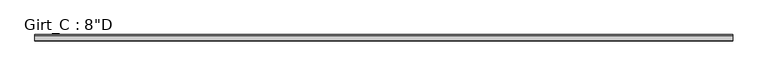
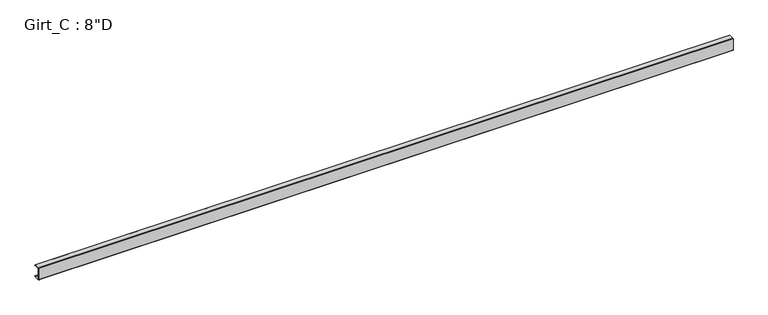
"""IFC4 building model written with IfcOpenShell, lengths in millimetres: beam geometry."""

from ifc_helpers import new_model, si_unit, point, frame, frame_2d, origin, place, context, project, spatial, polyline, circle_curve, trimmed, segment, composite_curve, outline, extrude, source, transform, mapped, element, save


def beam_732115ab(model_context):
    return source(origin(), model_context, "Body", "SweptSolid", [
        extrude(outline(composite_curve([segment(polyline([(87.5109375, 101.6), (99.7560415, 87.0068534), (97.6278742, 85.221109), (86.2154765, 98.821875), (3.3005807, 98.821875)]), True, "CONTINUOUS"), segment(trimmed(circle_curve(frame_2d((3.3741066, 96.8381931)), 1.9850441), [point((3.3005807, 98.821875))], [point((1.3890625, 96.8381931))], True, "CARTESIAN"), True, "CONTINUOUS"), segment(polyline([(1.3890625, 96.8381931), (1.3890625, -96.8389339)]), True, "CONTINUOUS"), segment(trimmed(circle_curve(frame_2d((3.3748024, -96.8389339)), 1.9857399), [point((1.3890625, -96.8389339))], [point((3.2694106, -98.821875))], True, "CARTESIAN"), True, "CONTINUOUS"), segment(polyline([(3.2694106, -98.821875), (86.2154765, -98.821875), (97.6510975, -85.1934327), (99.7792647, -86.979177), (87.5109375, -101.6), (3.3734375, -101.6)]), True, "CONTINUOUS"), segment(trimmed(circle_curve(frame_2d((3.3734375, -96.8375)), 4.7625), [point((3.3734375, -101.6))], [point((-1.3890625, -96.8375))], False, "CARTESIAN"), True, "CONTINUOUS"), segment(polyline([(-1.3890625, -96.8375), (-1.3890625, 96.8375)]), True, "CONTINUOUS"), segment(trimmed(circle_curve(frame_2d((3.3734375, 96.8375)), 4.7625), [point((-1.3890625, 96.8375))], [point((3.3734375, 101.6))], False, "CARTESIAN"), True, "CONTINUOUS"), segment(polyline([(3.3734375, 101.6), (87.5109375, 101.6)]), True, "CONTINUOUS")], self_intersect=False)), frame((-5606.5994778, 0.0, 0.0), z_axis=(1.0, 0.0, 0.0), x_axis=(0.0, 1.0, 0.0)), (0.0, 0.0, 1.0), 11099.7911069),
    ])


if __name__ == "__main__":
    model = new_model("IFC4")
    model_context = context("Model", 3, world=origin())
    ifc_project = project(units=[si_unit("LENGTHUNIT", "METRE", prefix="MILLI")], contexts=[model_context])
    site = spatial("IfcSite", under=ifc_project)
    building = spatial("IfcBuilding", under=site)
    placement = place(None, origin())
    beam_shape = beam_732115ab(model_context)
    element("IfcBeam", 1, ObjectType="Girt_C : 8\"D", at=placement, inside=building, context=model_context, shape_type="MappedRepresentation", body=[
        mapped(beam_shape, transform((0.0, 0.0, 0.0), x_axis=(1.0, 0.0, 0.0), y_axis=(0.0, 1.0, 0.0), z_axis=(0.0, 0.0, 1.0))),
    ])
    save(model, "model.ifc")

# Revit data of these elements
# Type "Girt_C : 8\"D"
#   half leg = 0' - 1 3/4"
#   Web_Thickness = 0' - 0 7/64"
#   Length [instance default] = 10' - 0"
#   Leg_1 = 0' - 3 1/2"
#   Height = 0' - 8"
#   Structural Material [instance default] = none
# Element 1 (IfcBeam, "Girt_C : 8\"D")
#   Structural Material = GALVANIZED 'CEE' SECTION (8.0x3.5C - SEE STRUCT. DWGS)
#   Materials on its faces: "GALVANIZED 'CEE' SECTION (8.0x3.5C - SEE STRUCT. DWGS)"
# Materials
#   "GALVANIZED 'CEE' SECTION (8.0x3.5C - SEE STRUCT. DWGS)": class "Metal", colour RGB 137 146 153, transparency 0, Description = "Steel, mill finish", Cost = 0
